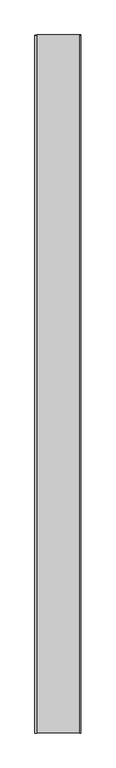
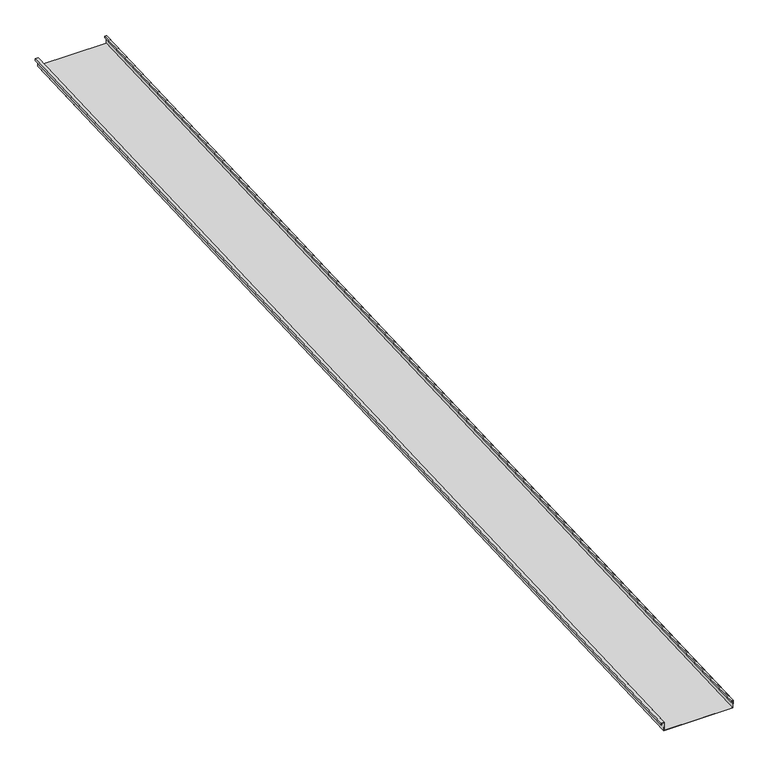
"""IFC4 building model written with IfcOpenShell, lengths in millimetres: proxy geometry, Generic Models 2:Generic Models 2:310765:Generic Models 2:310765 : Generic Models 2:Generic Models 2:310765:114 : Generic Models 2:Generic Models 2:310765:Generic Models 2:310765 : Generic Models 2:Generic Models 2:310765:300385."""

from ifc_helpers import new_model, si_unit, frame, origin, place, context, project, spatial, polyline, outline, extrude, source, transform, mapped, element, save


def generic_models_64278ea2(model_context):
    return source(origin(), model_context, "Body", "SweptSolid", [
        extrude(outline(polyline([(1.5875, 0.0), (1.5875, 50.8), (407.9875, 50.8), (407.9875, 1.5875), (396.875, 1.5875), (396.875, 11.1125), (398.4625, 11.1125), (398.4625, 3.175), (406.4, 3.175), (406.4, 49.2125), (3.175, 49.2125), (3.175, -1.5874999), (-14.2875, -1.5874999), (-14.2875, 9.525), (-12.7, 9.525), (-12.7, 0.0), (1.5875, 0.0)])), frame((666252.1763072, -581354.4345603, 3902.6697972), z_axis=(0.0, 0.9991330730923568, 0.041630544712067834), x_axis=(1.0, 0.0, 0.0)), (0.0, 0.0, 1.0), 6400.8),
    ])


if __name__ == "__main__":
    model = new_model("IFC4")
    model_context = context("Model", 3, world=origin())
    ifc_project = project(units=[si_unit("LENGTHUNIT", "METRE", prefix="MILLI")], contexts=[model_context])
    site = spatial("IfcSite", under=ifc_project)
    building = spatial("IfcBuilding", under=site)
    placement = place(None, origin())
    generic_models_shape = generic_models_64278ea2(model_context)
    element("IfcBuildingElementProxy", 1, Name="Generic Models 2:Generic Models 2:310765:Generic Models 2:310765 : Generic Models 2:Generic Models 2:310765:114 : Generic Models 2:Generic Models 2:310765:Generic Models 2:310765 : Generic Models 2:Generic Models 2:310765:300385", ObjectType="Generic Models 2:Generic Models 2:310765:Generic Models 2:310765 : Generic Models 2:Generic Models 2:310765:114 : Generic Models 2:Generic Models 2:310765:Generic Models 2:310765 : Generic Models 2:Generic Models 2:310765:300385", at=placement, inside=building, context=model_context, shape_type="MappedRepresentation", body=[
        mapped(generic_models_shape, transform((0.0, 0.0, 0.0), x_axis=(1.0, 0.0, 0.0), y_axis=(0.0, 1.0, 0.0), z_axis=(0.0, 0.0, 1.0))),
    ])
    save(model, "model.ifc")

# Revit data of these elements
# Type "Generic Models 2:Generic Models 2:310765:Generic Models 2:310765 : Generic Models 2:Generic Models 2:310765:114 : Generic Models 2:Generic Models 2:310765:Generic Models 2:310765 : Generic Models 2:Generic Models 2:310765:300385"
#   NameOverride = "Generic Models 2:Generic Models 2:310765:Generic Models 2:310765 : Generic Models 2:Generic Models 2:310765:300385"
#   ObjectTypeOverride = "Generic Models 2:310765 : Generic Models 2:Generic Models 2:310765"
#   Reference = "Generic Models 2"
#   Tag = "300385"
# Element 1 (IfcBuildingElementProxy, "Generic Models 2:Generic Models 2:310765:Generic Models 2:310765 : Generic Models 2:Generic Models 2:310765:114 : Generic Models 2:Generic Models 2:310765:Generic Models 2:310765 : Generic Models 2:Generic Models 2:310765:300385")
#   Materials on its faces: "THERMAL BROKEN ALUMINUM STOREFRONT FOR POLYCARBONATE"
# Materials
#   "THERMAL BROKEN ALUMINUM STOREFRONT FOR POLYCARBONATE": class "Unassigned", colour RGB 244 244 244, transparency 0, Keynote = "M07611300.01", Cost = 0
